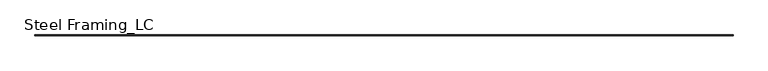
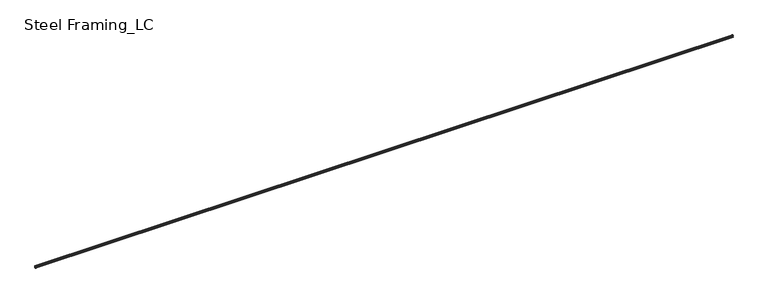
"""IFC4 building model written with IfcOpenShell, lengths in millimetres: beam geometry, Steel Framing_LC : H_SB_AR_S00_LC-150x75x25x3.2."""

from ifc_helpers import new_model, si_unit, point, frame, frame_2d, origin, place, context, project, spatial, polyline, circle_curve, trimmed, segment, composite_curve, outline, extrude, source, transform, mapped, element, save


def steel_framing_lc_58cf0942(model_context):
    return source(origin(), model_context, "Body", "SweptSolid", [
        extrude(outline(composite_curve([segment(polyline([(18.6, 67.0), (18.6, -67.0)]), True, "CONTINUOUS"), segment(trimmed(circle_curve(frame_2d((10.6, -67.0)), 8.0), [point((18.6, -67.0))], [point((10.6, -75.0))], False, "CARTESIAN"), True, "CONTINUOUS"), segment(polyline([(10.6, -75.0), (-48.4, -75.0)]), True, "CONTINUOUS"), segment(trimmed(circle_curve(frame_2d((-48.4, -67.0)), 8.0), [point((-48.4, -75.0))], [point((-56.4, -67.0))], False, "CARTESIAN"), True, "CONTINUOUS"), segment(polyline([(-56.4, -67.0), (-56.4, -50.0), (-53.2, -50.0), (-53.2, -67.0)]), True, "CONTINUOUS"), segment(trimmed(circle_curve(frame_2d((-48.4, -67.0)), 4.8), [point((-53.2, -67.0))], [point((-48.4, -71.8))], True, "CARTESIAN"), True, "CONTINUOUS"), segment(polyline([(-48.4, -71.8), (10.6, -71.8)]), True, "CONTINUOUS"), segment(trimmed(circle_curve(frame_2d((10.6, -67.0)), 4.8), [point((10.6, -71.8))], [point((15.4, -67.0))], True, "CARTESIAN"), True, "CONTINUOUS"), segment(polyline([(15.4, -67.0), (15.4, 67.0)]), True, "CONTINUOUS"), segment(trimmed(circle_curve(frame_2d((10.6, 67.0)), 4.8), [point((15.4, 67.0))], [point((10.6, 71.8))], True, "CARTESIAN"), True, "CONTINUOUS"), segment(polyline([(10.6, 71.8), (-48.4, 71.8)]), True, "CONTINUOUS"), segment(trimmed(circle_curve(frame_2d((-48.4, 67.0)), 4.8), [point((-48.4, 71.8))], [point((-53.2, 67.0))], True, "CARTESIAN"), True, "CONTINUOUS"), segment(polyline([(-53.2, 67.0), (-53.2, 50.0), (-56.4, 50.0), (-56.4, 67.0)]), True, "CONTINUOUS"), segment(trimmed(circle_curve(frame_2d((-48.4, 67.0)), 8.0), [point((-56.4, 67.0))], [point((-48.4, 75.0))], False, "CARTESIAN"), True, "CONTINUOUS"), segment(polyline([(-48.4, 75.0), (10.6, 75.0)]), True, "CONTINUOUS"), segment(trimmed(circle_curve(frame_2d((10.6, 67.0)), 8.0), [point((10.6, 75.0))], [point((18.6, 67.0))], False, "CARTESIAN"), True, "CONTINUOUS")], self_intersect=False)), frame((-30297.0, 0.0, 0.0), z_axis=(1.0, 0.0, 0.0), x_axis=(0.0, 1.0, 0.0)), (0.0, 0.0, 1.0), 60581.0),
    ])


if __name__ == "__main__":
    model = new_model("IFC4")
    model_context = context("Model", 3, world=origin())
    ifc_project = project(units=[si_unit("LENGTHUNIT", "METRE", prefix="MILLI")], contexts=[model_context])
    site = spatial("IfcSite", under=ifc_project)
    building = spatial("IfcBuilding", under=site)
    placement = place(None, origin())
    steel_framing_lc_shape = steel_framing_lc_58cf0942(model_context)
    element("IfcBeam", 1, ObjectType="Steel Framing_LC : H_SB_AR_S00_LC-150x75x25x3.2", at=placement, inside=building, context=model_context, shape_type="MappedRepresentation", body=[
        mapped(steel_framing_lc_shape, transform((0.0, 0.0, 0.0), x_axis=(1.0, 0.0, 0.0), y_axis=(0.0, 1.0, 0.0), z_axis=(0.0, 0.0, 1.0))),
    ])
    save(model, "model.ifc")

# Revit data of these elements
# Type "Steel Framing_LC : H_SB_AR_S00_LC-150x75x25x3.2"
#   Type Comments = "SECONDARY"
#   Type Mark = "GIRTH"
#   H_SectionID = "LC-150x75x25x3.2"
#   r = 4.8 mm
#   d = 25 mm
#   R = 8 mm
#   Perimeter = 0.70 m²/m
#   Nominal Weight = 10.30 kgf/m
#   Length [instance default] = 1000 mm
#   b = 75 mm
#   h = 150 mm
#   tw = 3.2 mm
#   x = 18.6 mm
#   A = 1.00 m²
#   Structural Material [instance default] = Steel, 45-345
#   Assembly Code = ""
# Element 1 (IfcBeam, "Steel Framing_LC : H_SB_AR_S00_LC-150x75x25x3.2")
#   Materials on its faces: "Steel, 45-345"
# Materials
#   "Steel, 45-345": class "Metal", colour RGB 189 187 185, transparency 0, Description = "Steel 345 MPa", Cost = 0
